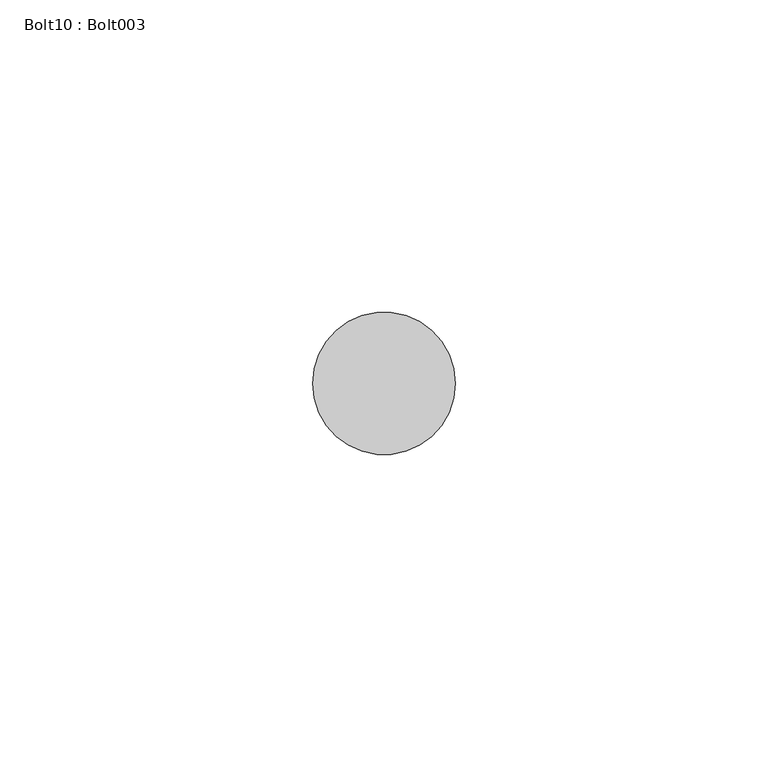
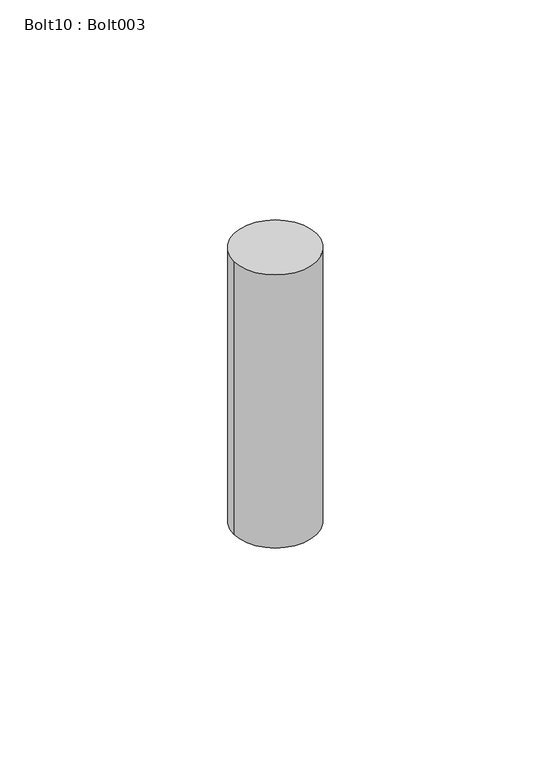
"""IFC4 building model written with IfcOpenShell, lengths in millimetres: proxy geometry, Bolt10 : Bolt003."""

from ifc_helpers import new_model, si_unit, point, frame, frame_2d, origin, place, context, project, spatial, circle_curve, trimmed, segment, composite_curve, outline, extrude, source, transform, mapped, element, save


def bolt10_bolt003_296b5833(model_context):
    return source(origin(), model_context, "Body", "SweptSolid", [
        extrude(outline(composite_curve([segment(trimmed(circle_curve(frame_2d((5172.3828124, 1998.1882072)), 11.4045168), [point((5160.9782956, 1998.1882072))], [point((5183.7873292, 1998.1882072))], False, "CARTESIAN"), True, "CONTINUOUS"), segment(trimmed(circle_curve(frame_2d((5172.3828124, 1998.1882072)), 11.4045168), [point((5183.7873292, 1998.1882072))], [point((5160.9782956, 1998.1882072))], False, "CARTESIAN"), True, "CONTINUOUS")], self_intersect=False)), frame((0.0, 0.0, 36645.5959962), z_axis=(0.0, 0.0, 1.0), x_axis=(1.0, 0.0, 0.0)), (0.0, 0.0, 1.0), 79.375),
    ])


if __name__ == "__main__":
    model = new_model("IFC4")
    model_context = context("Model", 3, world=origin())
    ifc_project = project(units=[si_unit("LENGTHUNIT", "METRE", prefix="MILLI")], contexts=[model_context])
    site = spatial("IfcSite", under=ifc_project)
    building = spatial("IfcBuilding", under=site)
    placement = place(None, origin())
    bolt10_bolt003_shape = bolt10_bolt003_296b5833(model_context)
    element("IfcBuildingElementProxy", 1, Name="Bolt10 : Bolt003", ObjectType="Bolt10 : Bolt003", at=placement, inside=building, context=model_context, shape_type="MappedRepresentation", body=[
        mapped(bolt10_bolt003_shape, transform((0.0, 0.0, 0.0), x_axis=(1.0, 0.0, 0.0), y_axis=(0.0, 1.0, 0.0), z_axis=(0.0, 0.0, 1.0))),
    ])
    save(model, "model.ifc")

# Revit data of these elements
# Type "Bolt10 : Bolt003"
#   NameOverride = "Bolt003"
# Element 1 (IfcBuildingElementProxy, "Bolt10 : Bolt003")
#   Materials on its faces: "TUBE STEEL STRINGER WELDED TO ANCHORED STEEL PLATE - SEE STRUCT DWGS"
# Materials
#   "TUBE STEEL STRINGER WELDED TO ANCHORED STEEL PLATE - SEE STRUCT DWGS": class "Unassigned", colour RGB 128 128 128, transparency 0, Cost = 0
